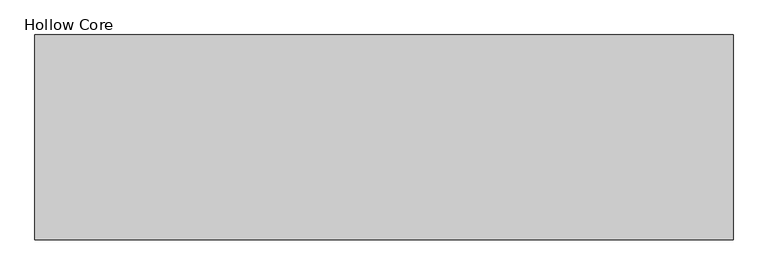
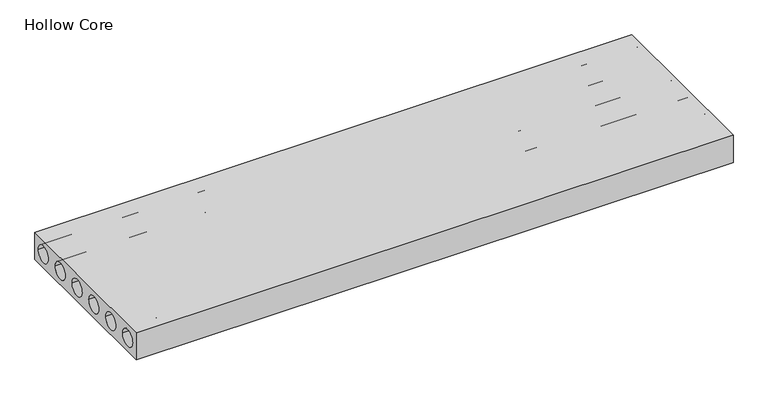
"""IFC4 building model written with IfcOpenShell, lengths in millimetres: proxy geometry, Hollow Core : Breton Hollow Core."""

from ifc_helpers import new_model, si_unit, point, frame, frame_2d, origin, place, context, project, spatial, polyline, circle_curve, trimmed, segment, composite_curve, outline, extrude, source, transform, mapped, element, save


def hollow_core_a6975cb3(model_context):
    return source(origin(), model_context, "Body", "SweptSolid", [
        extrude(outline(polyline([(-609.6, 100.0), (609.6, 100.0), (609.6, -100.0), (-609.6, -100.0), (-609.6, 100.0)]), holes=[composite_curve([segment(trimmed(circle_curve(frame_2d((508.0, 0.0)), 60.0), [point((448.0, 0.0))], [point((568.0, 0.0))], True, "CARTESIAN"), True, "CONTINUOUS"), segment(trimmed(circle_curve(frame_2d((508.0, 0.0)), 60.0), [point((568.0, 0.0))], [point((448.0, 0.0))], True, "CARTESIAN"), True, "CONTINUOUS")], self_intersect=False), composite_curve([segment(trimmed(circle_curve(frame_2d((-508.0, 0.0)), 60.0), [point((-568.0, 0.0))], [point((-448.0, 0.0))], True, "CARTESIAN"), True, "CONTINUOUS"), segment(trimmed(circle_curve(frame_2d((-508.0, 0.0)), 60.0), [point((-448.0, 0.0))], [point((-568.0, 0.0))], True, "CARTESIAN"), True, "CONTINUOUS")], self_intersect=False), composite_curve([segment(trimmed(circle_curve(frame_2d((304.8, 0.0)), 60.0), [point((244.8, 0.0))], [point((364.8, 0.0))], True, "CARTESIAN"), True, "CONTINUOUS"), segment(trimmed(circle_curve(frame_2d((304.8, 0.0)), 60.0), [point((364.8, 0.0))], [point((244.8, 0.0))], True, "CARTESIAN"), True, "CONTINUOUS")], self_intersect=False), composite_curve([segment(trimmed(circle_curve(frame_2d((101.6, 0.0)), 60.0), [point((41.6, 0.0))], [point((161.6, 0.0))], True, "CARTESIAN"), True, "CONTINUOUS"), segment(trimmed(circle_curve(frame_2d((101.6, 0.0)), 60.0), [point((161.6, 0.0))], [point((41.6, 0.0))], True, "CARTESIAN"), True, "CONTINUOUS")], self_intersect=False), composite_curve([segment(trimmed(circle_curve(frame_2d((-101.6, 0.0)), 60.0), [point((-161.6, 0.0))], [point((-41.6, 0.0))], True, "CARTESIAN"), True, "CONTINUOUS"), segment(trimmed(circle_curve(frame_2d((-101.6, 0.0)), 60.0), [point((-41.6, 0.0))], [point((-161.6, 0.0))], True, "CARTESIAN"), True, "CONTINUOUS")], self_intersect=False), composite_curve([segment(trimmed(circle_curve(frame_2d((-304.8, 0.0)), 60.0), [point((-364.8, 0.0))], [point((-244.8, 0.0))], True, "CARTESIAN"), True, "CONTINUOUS"), segment(trimmed(circle_curve(frame_2d((-304.8, 0.0)), 60.0), [point((-244.8, 0.0))], [point((-364.8, 0.0))], True, "CARTESIAN"), True, "CONTINUOUS")], self_intersect=False)]), frame((0.0, 0.0, 0.0), z_axis=(1.0, 0.0, 0.0), x_axis=(0.0, 1.0, 0.0)), (0.0, 0.0, 1.0), 4157.5),
    ])


if __name__ == "__main__":
    model = new_model("IFC4")
    model_context = context("Model", 3, world=origin())
    ifc_project = project(units=[si_unit("LENGTHUNIT", "METRE", prefix="MILLI")], contexts=[model_context])
    site = spatial("IfcSite", under=ifc_project)
    building = spatial("IfcBuilding", under=site)
    placement = place(None, origin())
    hollow_core_shape = hollow_core_a6975cb3(model_context)
    element("IfcBuildingElementProxy", 1, Name="Hollow Core : Breton Hollow Core", ObjectType="Hollow Core : Breton Hollow Core", at=placement, inside=building, context=model_context, shape_type="MappedRepresentation", body=[
        mapped(hollow_core_shape, transform((0.0, 0.0, 0.0), x_axis=(1.0, 0.0, 0.0), y_axis=(0.0, 1.0, 0.0), z_axis=(0.0, 0.0, 1.0))),
    ])
    save(model, "model.ifc")

# Revit data of these elements
# Type "Hollow Core : Breton Hollow Core"
#   Width [instance default] = 1219.2 mm
#   built-in parameter 1001306 [instance default] = 4 (stored number, unit not read)
#   Depth [instance default] = 152.4 mm
#   Core Radius [instance default] = 50.8 mm
#   Core Offset [instance default] = 101.6 mm
#   Number Of Cores [instance default] = 2
#   Material [instance default] = Concrete - Precast Concrete - Normal Weight - 5 ksi
#   Default Elevation = 0
#   Assembly Code = ""
# Element 1 (IfcBuildingElementProxy, "Hollow Core : Breton Hollow Core")
#   built-in parameter 1001306 = 13.6401 (stored number, unit not read)
#   Depth = 200 mm
#   Core Radius = 60 mm
#   Number Of Cores = 6
#   Materials on its faces: "Concrete - Precast Concrete - Normal Weight - 5 ksi"
# Materials
#   "Concrete - Precast Concrete - Normal Weight - 5 ksi": class "Concrete", colour RGB 198 187 187, transparency 0
